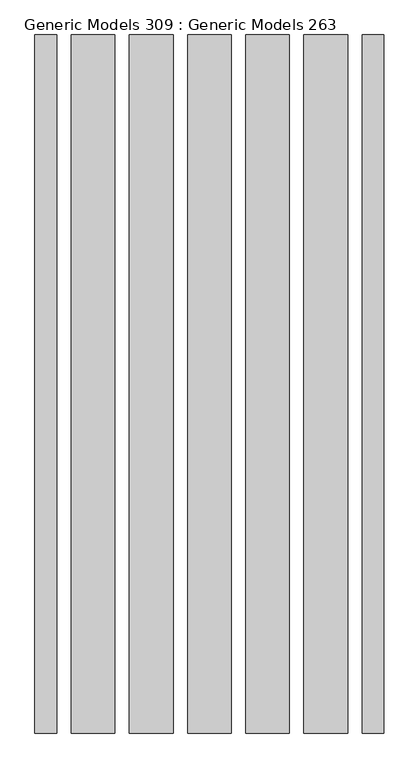
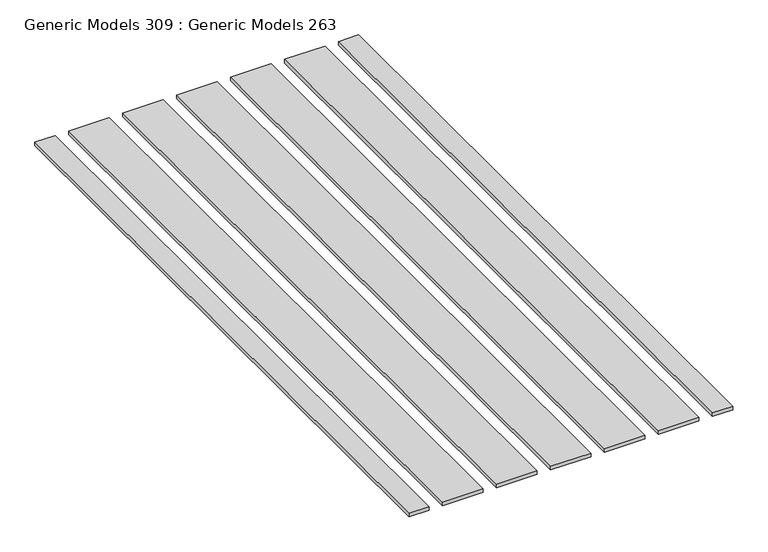
"""IFC4 building model written with IfcOpenShell, lengths in millimetres: proxy geometry, Generic Models 309 : Generic Models 263."""

from ifc_helpers import new_model, si_unit, frame, origin, place, context, project, spatial, polyline, outline, extrude, source, transform, mapped, element, save


def generic_models_309_generic_models_263_71f93402(model_context):
    return source(origin(), model_context, "Body", "SweptSolid", [
        extrude(outline(polyline([(94945.4797726, -94.4486541), (94907.3797726, -94.4486541), (94907.3797726, 1124.7513459), (94945.4797726, 1124.7513459), (94945.4797726, -94.4486541)])), frame((0.0, 0.0, -114.3), z_axis=(0.0, 0.0, 1.0), x_axis=(1.0, 0.0, 0.0)), (0.0, 0.0, 1.0), 7.0017153),
        extrude(outline(polyline([(95516.9797726, -94.4486541), (95478.8797726, -94.4486541), (95478.8797726, 1124.7513459), (95516.9797726, 1124.7513459), (95516.9797726, -94.4486541)])), frame((0.0, 0.0, -114.3), z_axis=(0.0, 0.0, 1.0), x_axis=(1.0, 0.0, 0.0)), (0.0, 0.0, 1.0), 7.0017153),
        extrude(outline(polyline([(95047.0797726, -94.4486541), (94970.8797726, -94.4486541), (94970.8797726, 1124.7513459), (95047.0797726, 1124.7513459), (95047.0797726, -94.4486541)])), frame((0.0, 0.0, -114.3), z_axis=(0.0, 0.0, 1.0), x_axis=(1.0, 0.0, 0.0)), (0.0, 0.0, 1.0), 7.0017153),
        extrude(outline(polyline([(95148.6797726, -94.4486541), (95072.4797726, -94.4486541), (95072.4797726, 1124.7513459), (95148.6797726, 1124.7513459), (95148.6797726, -94.4486541)])), frame((0.0, 0.0, -114.3), z_axis=(0.0, 0.0, 1.0), x_axis=(1.0, 0.0, 0.0)), (0.0, 0.0, 1.0), 7.0017153),
        extrude(outline(polyline([(95250.2797726, -94.4486541), (95174.0797726, -94.4486541), (95174.0797726, 1124.7513459), (95250.2797726, 1124.7513459), (95250.2797726, -94.4486541)])), frame((0.0, 0.0, -114.3), z_axis=(0.0, 0.0, 1.0), x_axis=(1.0, 0.0, 0.0)), (0.0, 0.0, 1.0), 7.0017153),
        extrude(outline(polyline([(95351.8797726, -94.4486541), (95275.6797726, -94.4486541), (95275.6797726, 1124.7513459), (95351.8797726, 1124.7513459), (95351.8797726, -94.4486541)])), frame((0.0, 0.0, -114.3), z_axis=(0.0, 0.0, 1.0), x_axis=(1.0, 0.0, 0.0)), (0.0, 0.0, 1.0), 7.0017153),
        extrude(outline(polyline([(95453.4797726, -94.4486541), (95377.2797726, -94.4486541), (95377.2797726, 1124.7513459), (95453.4797726, 1124.7513459), (95453.4797726, -94.4486541)])), frame((0.0, 0.0, -114.3), z_axis=(0.0, 0.0, 1.0), x_axis=(1.0, 0.0, 0.0)), (0.0, 0.0, 1.0), 7.0017153),
    ])


if __name__ == "__main__":
    model = new_model("IFC4")
    model_context = context("Model", 3, world=origin())
    ifc_project = project(units=[si_unit("LENGTHUNIT", "METRE", prefix="MILLI")], contexts=[model_context])
    site = spatial("IfcSite", under=ifc_project)
    building = spatial("IfcBuilding", under=site)
    placement = place(None, origin())
    generic_models_309_generic_models_263_shape = generic_models_309_generic_models_263_71f93402(model_context)
    element("IfcBuildingElementProxy", 1, Name="Generic Models 309 : Generic Models 263", ObjectType="Generic Models 309 : Generic Models 263", at=placement, inside=building, context=model_context, shape_type="MappedRepresentation", body=[
        mapped(generic_models_309_generic_models_263_shape, transform((0.0, 0.0, 0.0), x_axis=(1.0, 0.0, 0.0), y_axis=(0.0, 1.0, 0.0), z_axis=(0.0, 0.0, 1.0))),
    ])
    save(model, "model.ifc")

# Revit data of these elements
# Element 1 (IfcBuildingElementProxy, "Generic Models 309 : Generic Models 263")
#   Materials on its faces: "EPOXY COATED 6 X 6 X W2.9 X W2.9, PLACED 3\" ABOVE SLAB BASE"
# Materials
#   "EPOXY COATED 6 X 6 X W2.9 X W2.9, PLACED 3\" ABOVE SLAB BASE": class "Miscellaneous", colour RGB 44 44 44, transparency 0, Cost = 0
